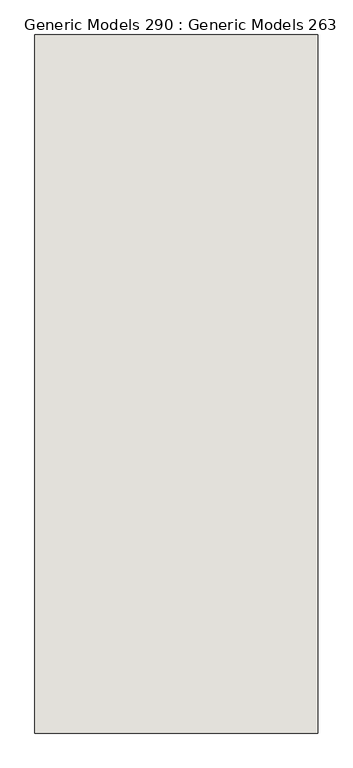
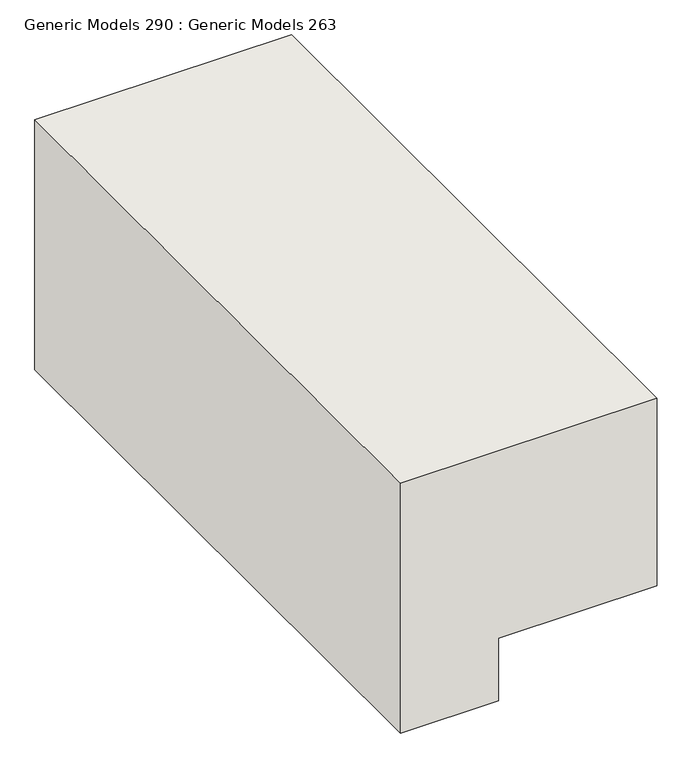
"""IFC4 building model written with IfcOpenShell, lengths in millimetres: wall geometry, Generic Models 290 : Generic Models 263."""

from ifc_helpers import new_model, si_unit, frame, origin, place, context, project, spatial, polyline, outline, extrude, source, transform, mapped, element, save


def generic_models_290_generic_models_263_8c817db6(model_context):
    return source(origin(), model_context, "Body", "SweptSolid", [
        extrude(outline(polyline([(-381.0, 60490.3797726), (0.0, 60490.3797726), (0.0, 59996.6389907), (-508.0, 59996.6389907), (-508.0, 60185.5797726), (-381.0, 60185.5797726), (-381.0, 60490.3797726)])), frame((0.0, -94.4486541, 0.0), z_axis=(0.0, 1.0, 0.0), x_axis=(0.0, 0.0, 1.0)), (0.0, 0.0, 1.0), 1219.2),
    ])


if __name__ == "__main__":
    model = new_model("IFC4")
    model_context = context("Model", 3, world=origin())
    ifc_project = project(units=[si_unit("LENGTHUNIT", "METRE", prefix="MILLI")], contexts=[model_context])
    site = spatial("IfcSite", under=ifc_project)
    building = spatial("IfcBuilding", under=site)
    placement = place(None, origin())
    generic_models_290_generic_models_263_shape = generic_models_290_generic_models_263_8c817db6(model_context)
    element("IfcWall", 1, ObjectType="Generic Models 290 : Generic Models 263", at=placement, inside=building, context=model_context, shape_type="MappedRepresentation", body=[
        mapped(generic_models_290_generic_models_263_shape, transform((0.0, 0.0, 0.0), x_axis=(1.0, 0.0, 0.0), y_axis=(0.0, 1.0, 0.0), z_axis=(0.0, 0.0, 1.0))),
    ])
    save(model, "model.ifc")

# Revit data of these elements
# Element 1 (IfcWall, "Generic Models 290 : Generic Models 263")
#   Materials on its faces: "GRADED BACKFILL"
# Materials
#   "GRADED BACKFILL": class "Miscellaneous", colour RGB 128 97 77, transparency 0, Cost = 0
